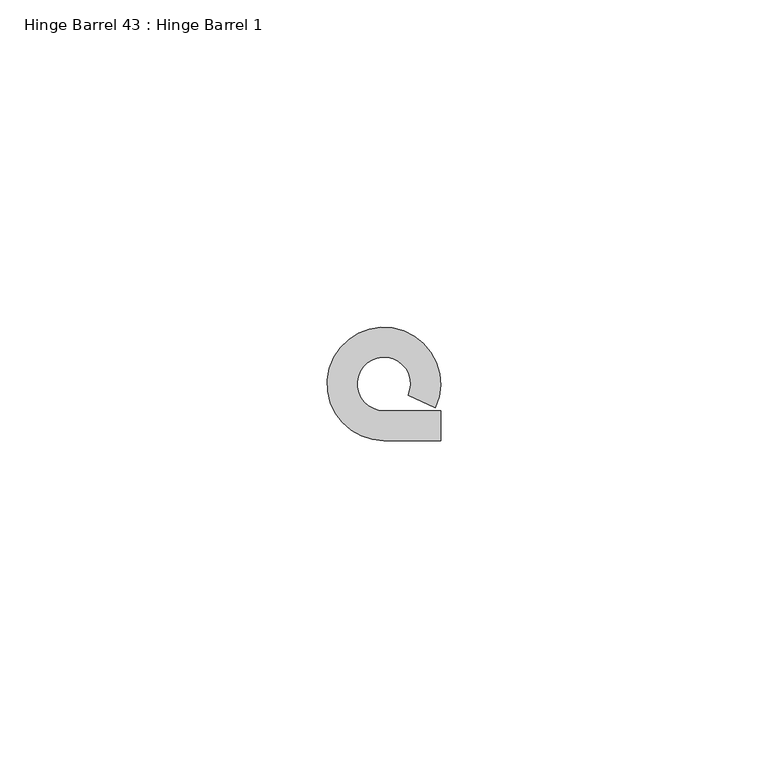
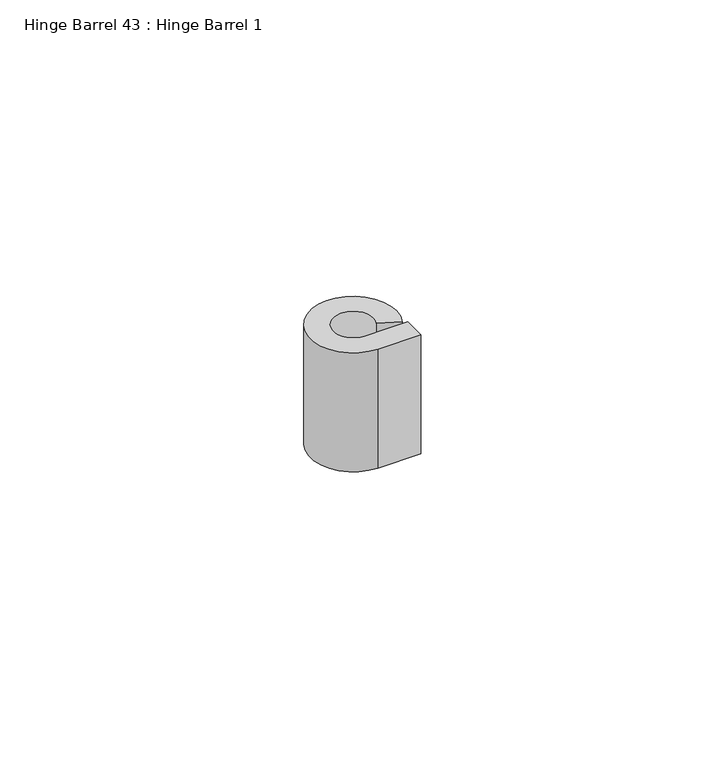
"""IFC4 building model written with IfcOpenShell, lengths in millimetres: proxy geometry, Hinge Barrel 43 : Hinge Barrel 1."""

from ifc_helpers import new_model, si_unit, point, frame, frame_2d, origin, place, context, project, spatial, polyline, circle_curve, trimmed, segment, composite_curve, outline, extrude, source, transform, mapped, element, save


def hinge_barrel_43_hinge_barrel_1_81794a76(model_context):
    return source(origin(), model_context, "Body", "SweptSolid", [
        extrude(outline(composite_curve([segment(polyline([(587323.2214739, -534104.7943841), (587327.7934739, -534104.7943841), (587327.7934739, -534109.3584466), (587319.1320739, -534109.3584466)]), True, "CONTINUOUS"), segment(trimmed(circle_curve(frame_2d((587319.1320739, -534100.7049841)), 8.6534625), [point((587319.1320739, -534109.3584466))], [point((587326.986084, -534104.3377433))], False, "CARTESIAN"), True, "CONTINUOUS"), segment(polyline([(587326.986084, -534104.3377433), (587322.8436736, -534102.421731)]), True, "CONTINUOUS"), segment(trimmed(circle_curve(frame_2d((587319.1320739, -534100.7049841)), 4.0894), [point((587322.8436736, -534102.421731))], [point((587319.1320739, -534104.7943841))], True, "CARTESIAN"), True, "CONTINUOUS"), segment(polyline([(587319.1320739, -534104.7943841), (587323.2214739, -534104.7943841)]), True, "CONTINUOUS")], self_intersect=False)), frame((0.0, 0.0, 1936.75), z_axis=(0.0, 0.0, 1.0), x_axis=(1.0, 0.0, 0.0)), (0.0, 0.0, 1.0), 25.4),
    ])


if __name__ == "__main__":
    model = new_model("IFC4")
    model_context = context("Model", 3, world=origin())
    ifc_project = project(units=[si_unit("LENGTHUNIT", "METRE", prefix="MILLI")], contexts=[model_context])
    site = spatial("IfcSite", under=ifc_project)
    building = spatial("IfcBuilding", under=site)
    placement = place(None, origin())
    hinge_barrel_43_hinge_barrel_1_shape = hinge_barrel_43_hinge_barrel_1_81794a76(model_context)
    element("IfcBuildingElementProxy", 1, Name="Hinge Barrel 43 : Hinge Barrel 1", ObjectType="Hinge Barrel 43 : Hinge Barrel 1", at=placement, inside=building, context=model_context, shape_type="MappedRepresentation", body=[
        mapped(hinge_barrel_43_hinge_barrel_1_shape, transform((0.0, 0.0, 0.0), x_axis=(1.0, 0.0, 0.0), y_axis=(0.0, 1.0, 0.0), z_axis=(0.0, 0.0, 1.0))),
    ])
    save(model, "model.ifc")

# Revit data of these elements
# Element 1 (IfcBuildingElementProxy, "Hinge Barrel 43 : Hinge Barrel 1")
#   Materials on its faces: "6\"X6\" WELD-ON STL BUTT HINGE"
# Materials
#   "6\"X6\" WELD-ON STL BUTT HINGE": class "Metal", colour RGB 189 187 185, transparency 0, Description = "Carbon steel", Cost = 0
